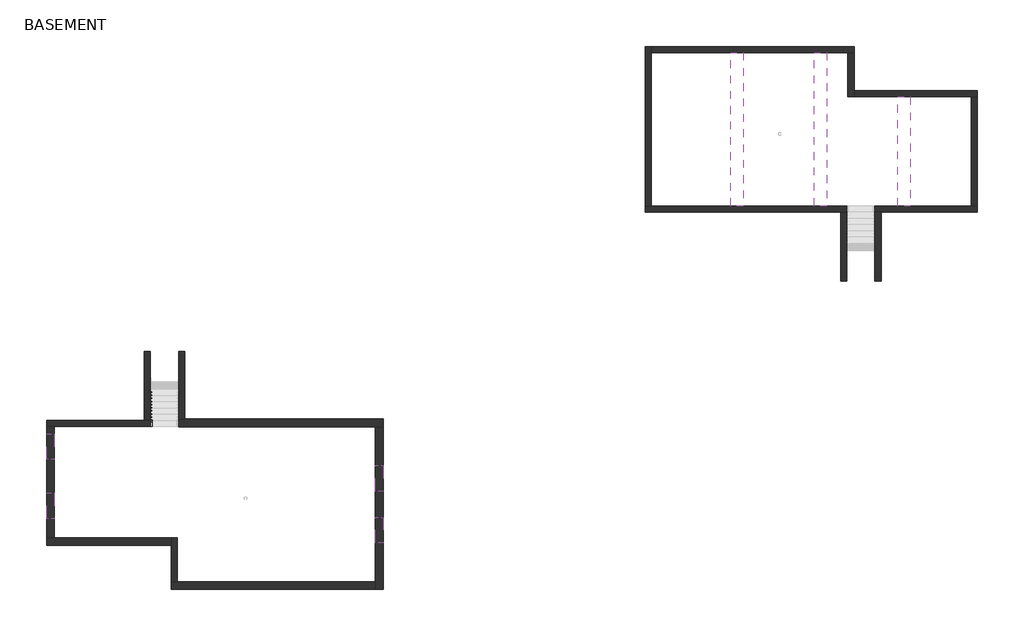
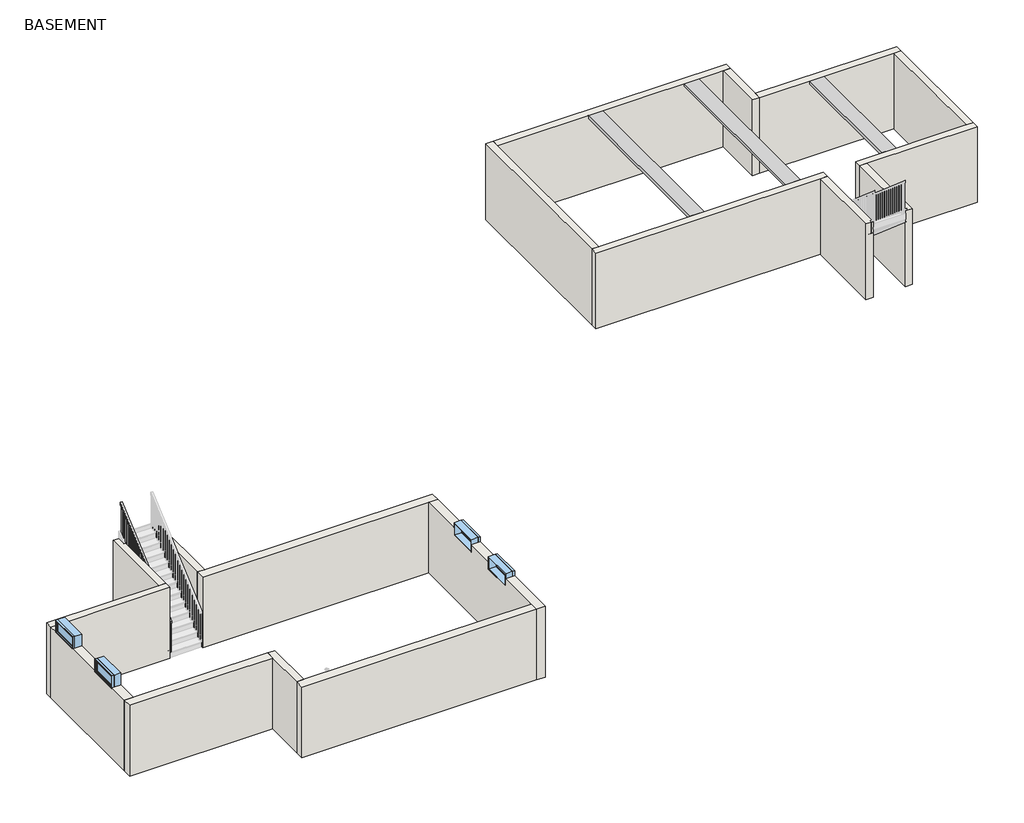
# One storey, part 1 of 2: 18 walls, 4 windows, 3 beams, 1 railing.
"""IFC4 building model written with IfcOpenShell, lengths in millimetres."""

import ifcopenshell
import ifcopenshell.guid

model = None  # the IFC model being written
_history = None  # IfcOwnerHistory: only IFC2X3 demands one
_inside = {}  # id of a spatial element -> (the spatial element, [elements in it])
_under = {}  # id of a project, library or spatial element -> (it, [spatial elements below it])
_declared = {}  # id of a project -> (the project, [libraries it declares])
_typed = {}  # id of a type object -> (the type object, [elements of that type])
_made_of = {}  # id of a material, layer set ... -> (it, [elements and type objects made of it])


def new_model(schema):
    """Start an empty IFC model of exactly this schema.

    Asked for "IFC4X3", IfcOpenShell would pick the latest addendum, in which some entities
    have other attributes; the version numbers below select the first issue.
    IFC2X3 requires an IfcOwnerHistory on every rooted entity: one is made here for all.
    """
    global model, _history
    if schema == "IFC4X3":
        model = ifcopenshell.file(schema_version=(4, 3, 0, 0))
    else:
        model = ifcopenshell.file(schema=schema)
    _inside.clear()
    _under.clear()
    _declared.clear()
    _typed.clear()
    _made_of.clear()
    _history = None
    if model.schema == "IFC2X3":
        org = make("IfcOrganization", Name="unknown")
        user = make(
            "IfcPersonAndOrganization",
            ThePerson=make("IfcPerson", FamilyName="unknown"),
            TheOrganization=org,
        )
        app = make(
            "IfcApplication",
            ApplicationDeveloper=org,
            Version="unknown",
            ApplicationFullName="unknown",
            ApplicationIdentifier="unknown",
        )
        _history = make(
            "IfcOwnerHistory",
            OwningUser=user,
            OwningApplication=app,
            ChangeAction="ADDED",
            CreationDate=0,
        )
    return model


def make(cls, **values):
    """One entity of the class cls with the attributes given. An attribute that is None is left unset."""
    return model.create_entity(
        cls, **{name: value for name, value in values.items() if value is not None}
    )


def rooted(cls, **values):
    """An entity with a GlobalId (a new one), such as an element, a storey or a relation."""
    return make(cls, GlobalId=ifcopenshell.guid.new(), OwnerHistory=_history, **values)


def si_unit(unit_type, name, prefix=None):
    """IfcSIUnit, for example si_unit("LENGTHUNIT", "METRE", prefix="MILLI")."""
    return make("IfcSIUnit", UnitType=unit_type, Prefix=prefix, Name=name)


def assignment(units):
    """IfcUnitAssignment: the units of a project."""
    return None if units is None else make("IfcUnitAssignment", Units=units)


def point(xyz):
    """IfcCartesianPoint."""
    return None if xyz is None else make("IfcCartesianPoint", Coordinates=xyz)


def direction(xyz):
    """IfcDirection."""
    return None if xyz is None else make("IfcDirection", DirectionRatios=xyz)


def frame(location, z_axis=None, x_axis=None):
    """IfcAxis2Placement3D, a coordinate frame: its origin and axes. An axis left out is left unset."""
    return make(
        "IfcAxis2Placement3D",
        Location=point(location),
        Axis=direction(z_axis),
        RefDirection=direction(x_axis),
    )


def origin():
    """The frame at (0, 0, 0) with its axes left unset."""
    return frame((0.0, 0.0, 0.0))


def place(relative_to, where):
    """IfcLocalPlacement: puts the frame where relative to a parent placement (None: the world)."""
    return make(
        "IfcLocalPlacement", PlacementRelTo=relative_to, RelativePlacement=where
    )


def context(
    kind, dimensions, precision=None, world=None, true_north=None, identifier=None
):
    """IfcGeometricRepresentationContext, for example the 3D "Model" context."""
    return make(
        "IfcGeometricRepresentationContext",
        ContextIdentifier=identifier,
        ContextType=kind,
        CoordinateSpaceDimension=dimensions,
        Precision=precision,
        WorldCoordinateSystem=world,
        TrueNorth=true_north,
    )


def project(units=None, contexts=None):
    """IfcProject with its units and contexts."""
    return rooted(
        "IfcProject",
        Name="project",
        RepresentationContexts=contexts,
        UnitsInContext=assignment(units),
    )


def spatial(cls, under=None, at=None, **own):
    """A site, building, storey or space (cls), placed at a placement, below another one or the project."""
    s = rooted(cls, ObjectPlacement=at, **own)
    if under is not None:
        _under.setdefault(under.id(), (under, []))[1].append(s)
    return s


def polyline(points):
    """IfcPolyline through the points."""
    return make("IfcPolyline", Points=[point(p) for p in points])


def outline(outer, holes=None, kind="AREA"):
    """IfcArbitraryClosedProfileDef: a profile drawn as a closed curve; with holes, ...WithVoids."""
    if holes is None:
        return make("IfcArbitraryClosedProfileDef", ProfileType=kind, OuterCurve=outer)
    return make(
        "IfcArbitraryProfileDefWithVoids",
        ProfileType=kind,
        OuterCurve=outer,
        InnerCurves=holes,
    )


def extrude(swept, where, along, depth):
    """IfcExtrudedAreaSolid: the profile swept, set in the frame where, extruded along a direction by depth."""
    return make(
        "IfcExtrudedAreaSolid",
        SweptArea=swept,
        Position=where,
        ExtrudedDirection=direction(along),
        Depth=depth,
    )


def faces_of(points, faces, orient=None, outer=None):
    """IfcFace entities. A face is a list of loops; a loop is a list of indices into points, from 0.

    orient and outer hold one flag for each loop. By default every Orientation is true, the
    first loop of a face is its IfcFaceOuterBound and the others are IfcFaceBound.
    """
    made = []
    for i, loops in enumerate(faces):
        bounds = []
        for j, loop in enumerate(loops):
            is_outer = j == 0 if outer is None else outer[i][j]
            bounds.append(
                make(
                    "IfcFaceOuterBound" if is_outer else "IfcFaceBound",
                    Bound=make("IfcPolyLoop", Polygon=[points[k] for k in loop]),
                    Orientation=True if orient is None else orient[i][j],
                )
            )
        made.append(make("IfcFace", Bounds=bounds))
    return made


def faceted_brep(points, faces, orient=None, outer=None, voids=None):
    """IfcFacetedBrep: a solid bounded by flat faces; with voids (closed shells), ...WithVoids."""
    shared = [point(p) for p in points]
    hull = make("IfcClosedShell", CfsFaces=faces_of(shared, faces, orient, outer))
    if voids is None:
        return make("IfcFacetedBrep", Outer=hull)
    return make(
        "IfcFacetedBrepWithVoids",
        Outer=hull,
        Voids=[
            make(cls, CfsFaces=faces_of(shared, fs, o, b)) for cls, fs, o, b in voids
        ],
    )


def shape(context_of_items, identifier, shape_type, items):
    """IfcShapeRepresentation: the items that make up one representation, for example the "Body"."""
    return make(
        "IfcShapeRepresentation",
        ContextOfItems=context_of_items,
        RepresentationIdentifier=identifier,
        RepresentationType=shape_type,
        Items=items,
    )


def source(mapping_origin, context_of_items, identifier, shape_type, items):
    """IfcRepresentationMap: a shape defined once, which mapped items show again and again."""
    return make(
        "IfcRepresentationMap",
        MappingOrigin=mapping_origin,
        MappedRepresentation=shape(context_of_items, identifier, shape_type, items),
    )


def transform(
    local_origin,
    x_axis=None,
    y_axis=None,
    z_axis=None,
    scale=None,
    scale2=None,
    scale3=None,
    uniform=True,
):
    """IfcCartesianTransformationOperator3D, or its non-uniform kind. x_axis, y_axis, z_axis: its Axis1, 2, 3."""
    if uniform:
        return make(
            "IfcCartesianTransformationOperator3D",
            Axis1=direction(x_axis),
            Axis2=direction(y_axis),
            LocalOrigin=point(local_origin),
            Scale=scale,
            Axis3=direction(z_axis),
        )
    return make(
        "IfcCartesianTransformationOperator3DnonUniform",
        Axis1=direction(x_axis),
        Axis2=direction(y_axis),
        LocalOrigin=point(local_origin),
        Scale=scale,
        Axis3=direction(z_axis),
        Scale2=scale2,
        Scale3=scale3,
    )


def mapped(mapping_source, mapping_target):
    """IfcMappedItem: shows the shape of a source again, moved by a transform."""
    return make(
        "IfcMappedItem", MappingSource=mapping_source, MappingTarget=mapping_target
    )


def made_of(thing, what):
    """Note that an element or type object is made of a material, layer set ...; save() writes the relation."""
    if what is not None:
        _made_of.setdefault(what.id(), (what, []))[1].append(thing)
    return thing


def element(
    cls,
    number,
    at=None,
    inside=None,
    cuts=None,
    type_object=None,
    material=None,
    context=None,
    identifier="Body",
    shape_type=None,
    held_by="IfcProductDefinitionShape",
    body=None,
    shapes=None,
    **own,
):
    """One element of the class cls, such as IfcWall. Its Tag is "e" and its number.

    at: its placement. inside: the storey or other place that contains it. cuts: it is an
    opening in that element (IfcRelVoidsElement). A single representation is given by context,
    identifier, shape_type and body (its items); several are given by shapes. held_by: the class
    of the entity that holds the representations. save() writes the other relations.
    """
    e = rooted(cls, Tag="e%d" % number, ObjectPlacement=at, **own)
    if body is not None:
        shapes = [shape(context, identifier, shape_type, body)]
    if shapes is not None:
        e.Representation = make(held_by, Representations=shapes)
    if inside is not None:
        _inside.setdefault(inside.id(), (inside, []))[1].append(e)
    if cuts is not None:
        rooted(
            "IfcRelVoidsElement", RelatingBuildingElement=cuts, RelatedOpeningElement=e
        )
    if type_object is not None:
        _typed.setdefault(type_object.id(), (type_object, []))[1].append(e)
    return made_of(e, material)


def aggregate(whole, parts):
    """IfcRelAggregates: a whole, such as a stair, and the parts it consists of."""
    return rooted("IfcRelAggregates", RelatingObject=whole, RelatedObjects=parts)


def save(model, path):
    """Write the relations noted so far, then the file.

    IfcRelAggregates (storeys below a building ...), IfcRelContainedInSpatialStructure (elements
    in a storey), IfcRelDefinesByType, IfcRelAssociatesMaterial and IfcRelDeclares: one each for
    every whole, place, type object, material and project.
    """
    for whole, parts in _under.values():
        aggregate(whole, parts)
    for where, things in _inside.values():
        rooted(
            "IfcRelContainedInSpatialStructure",
            RelatedElements=things,
            RelatingStructure=where,
        )
    for kind, things in _typed.values():
        rooted("IfcRelDefinesByType", RelatedObjects=things, RelatingType=kind)
    for what, things in _made_of.values():
        rooted("IfcRelAssociatesMaterial", RelatedObjects=things, RelatingMaterial=what)
    for by, libraries in _declared.values():
        rooted("IfcRelDeclares", RelatingContext=by, RelatedDefinitions=libraries)
    model.write(path)


def window_bf5cd34b(model_context):
    return source(origin(), model_context, "Body", "SweptSolid", [
        extrude(outline(polyline([(317.5, 79.375), (-393.7, 79.375), (-393.7, 92.075), (317.5, 92.075), (317.5, 79.375)])), frame((0.0, 0.0, 977.9), z_axis=(0.0, 0.0, 1.0), x_axis=(1.0, 0.0, 0.0)), (0.0, 0.0, 1.0), 254.0),
        extrude(outline(polyline([(1276.35, -438.15), (933.45, -438.15), (933.45, 361.95), (1276.35, 361.95), (1276.35, -438.15)]), holes=[polyline([(1231.9, -393.7), (1231.9, 317.5), (977.9, 317.5), (977.9, -393.7), (1231.9, -393.7)])]), frame((0.0, 63.5, 0.0), z_axis=(0.0, 1.0, 0.0), x_axis=(0.0, 0.0, 1.0)), (0.0, 0.0, 1.0), 44.45),
        extrude(outline(polyline([(1295.4, -457.2), (914.4, -457.2), (914.4, 381.0), (1295.4, 381.0), (1295.4, -457.2)]), holes=[polyline([(1263.65, -425.45), (1263.65, 349.25), (946.15, 349.25), (946.15, -425.45), (1263.65, -425.45)])]), frame((0.0, -127.0, 0.0), z_axis=(0.0, 1.0, 0.0), x_axis=(0.0, 0.0, 1.0)), (0.0, 0.0, 1.0), 190.5),
        extrude(outline(polyline([(1295.4, 381.0), (1295.4, -457.2), (914.4, -457.2), (914.4, 381.0), (1295.4, 381.0)]), holes=[polyline([(1276.35, 361.95), (933.45, 361.95), (933.45, -438.15), (1276.35, -438.15), (1276.35, 361.95)])]), frame((0.0, 63.5, 0.0), z_axis=(0.0, 1.0, 0.0), x_axis=(0.0, 0.0, 1.0)), (0.0, 0.0, 1.0), 63.5),
    ])


model = new_model("IFC4")

# Units and contexts
model_context = context("Model", 3, world=origin())
ifc_project = project(units=[si_unit("LENGTHUNIT", "METRE", prefix="MILLI")], contexts=[model_context])

# Site, building, storey
site = spatial("IfcSite", under=ifc_project)
building = spatial("IfcBuilding", under=site)
storey = spatial("IfcBuildingStorey", under=building, Name="BASEMENT", Elevation=-2266.95)

# Beams
placement = place(None, origin())
element("IfcBeam", 1, ObjectType="Concrete-Rectangular Beam : width=1' - 4\" x depth=0'  3 1/4\"", at=placement, inside=storey, context=model_context, shape_type="SweptSolid", body=[
    extrude(outline(polyline([(-3464.4595256, -410.4444564), (-3058.0595256, -410.4444564), (-3058.0595256, -5395.1944564), (-3464.4595256, -5395.1944564), (-3464.4595256, -410.4444564)])), frame((0.0, 0.0, -82.55), z_axis=(0.0, 0.0, 1.0), x_axis=(1.0, 0.0, 0.0)), (0.0, 0.0, 1.0), 82.55),
])
element("IfcBeam", 2, ObjectType="Concrete-Rectangular Beam : width=1' - 4\" x depth=0'  3 1/4\"", at=placement, inside=storey, context=model_context, shape_type="SweptSolid", body=[
    extrude(outline(polyline([(-6182.2595256, -410.4444564), (-5775.8595256, -410.4444564), (-5775.8595256, -5395.1944564), (-6182.2595256, -5395.1944564), (-6182.2595256, -410.4444564)])), frame((0.0, 0.0, -82.55), z_axis=(0.0, 0.0, 1.0), x_axis=(1.0, 0.0, 0.0)), (0.0, 0.0, 1.0), 82.55),
])
element("IfcBeam", 3, ObjectType="Concrete-Rectangular Beam : width=1' - 4\" x depth=0'  3 1/4\"", at=placement, inside=storey, context=model_context, shape_type="SweptSolid", body=[
    extrude(outline(polyline([(-746.6595256, -1845.5444564), (-340.2595256, -1845.5444564), (-340.2595256, -5395.1944564), (-746.6595256, -5395.1944564), (-746.6595256, -1845.5444564)])), frame((0.0, 0.0, -82.55), z_axis=(0.0, 0.0, 1.0), x_axis=(1.0, 0.0, 0.0)), (0.0, 0.0, 1.0), 82.55),
])

# Railing
element("IfcRailing", 4, ObjectType="Handrail - Rectangular", at=placement, inside=storey, context=model_context, shape_type="SweptSolid", body=[
    extrude(outline(polyline([(-12572.2570712, -1245.110853), (-12572.2570712, -1178.1692308), (-10133.8570712, 914.4), (-10133.8570712, 847.4583777), (-12572.2570712, -1245.110853)])), frame((-25042.4664763, 0.0, 0.0), z_axis=(1.0, 0.0, 0.0), x_axis=(0.0, 1.0, 0.0)), (0.0, 0.0, 1.0), 50.8),
    extrude(outline(polyline([(-10225.9320712, 768.4420917), (-10225.9320712, -174.3807692), (-10244.9820712, -174.3807692), (-10244.9820712, 752.0938946), (-10225.9320712, 768.4420917)])), frame((-25026.5914763, 0.0, 0.0), z_axis=(1.0, 0.0, 0.0), x_axis=(0.0, 1.0, 0.0)), (0.0, 0.0, 1.0), 19.05),
    extrude(outline(polyline([(-10327.5320712, 681.2517071), (-10327.5320712, -174.3807692), (-10346.5820712, -174.3807692), (-10346.5820712, 664.9035099), (-10327.5320712, 681.2517071)])), frame((-25026.5914763, 0.0, 0.0), z_axis=(1.0, 0.0, 0.0), x_axis=(0.0, 1.0, 0.0)), (0.0, 0.0, 1.0), 19.05),
    extrude(outline(polyline([(-10429.1320712, 594.0613224), (-10429.1320712, -348.7615385), (-10448.1820712, -348.7615385), (-10448.1820712, 577.7131253), (-10429.1320712, 594.0613224)])), frame((-25026.5914763, 0.0, 0.0), z_axis=(1.0, 0.0, 0.0), x_axis=(0.0, 1.0, 0.0)), (0.0, 0.0, 1.0), 19.05),
    extrude(outline(polyline([(-10530.7320712, 506.8709378), (-10530.7320712, -348.7615385), (-10549.7820712, -348.7615385), (-10549.7820712, 490.5227407), (-10530.7320712, 506.8709378)])), frame((-25026.5914763, 0.0, 0.0), z_axis=(1.0, 0.0, 0.0), x_axis=(0.0, 1.0, 0.0)), (0.0, 0.0, 1.0), 19.05),
    extrude(outline(polyline([(-10632.3320712, 419.6805532), (-10632.3320712, -523.1423077), (-10651.3820712, -523.1423077), (-10651.3820712, 403.3323561), (-10632.3320712, 419.6805532)])), frame((-25026.5914763, 0.0, 0.0), z_axis=(1.0, 0.0, 0.0), x_axis=(0.0, 1.0, 0.0)), (0.0, 0.0, 1.0), 19.05),
    extrude(outline(polyline([(-10733.9320712, 332.4901686), (-10733.9320712, -523.1423077), (-10752.9820712, -523.1423077), (-10752.9820712, 316.1419715), (-10733.9320712, 332.4901686)])), frame((-25026.5914763, 0.0, 0.0), z_axis=(1.0, 0.0, 0.0), x_axis=(0.0, 1.0, 0.0)), (0.0, 0.0, 1.0), 19.05),
    extrude(outline(polyline([(-10835.5320712, 245.299784), (-10835.5320712, -697.5230769), (-10854.5820712, -697.5230769), (-10854.5820712, 228.9515869), (-10835.5320712, 245.299784)])), frame((-25026.5914763, 0.0, 0.0), z_axis=(1.0, 0.0, 0.0), x_axis=(0.0, 1.0, 0.0)), (0.0, 0.0, 1.0), 19.05),
    extrude(outline(polyline([(-10937.1320712, 158.1093994), (-10937.1320712, -697.5230769), (-10956.1820712, -697.5230769), (-10956.1820712, 141.7612022), (-10937.1320712, 158.1093994)])), frame((-25026.5914763, 0.0, 0.0), z_axis=(1.0, 0.0, 0.0), x_axis=(0.0, 1.0, 0.0)), (0.0, 0.0, 1.0), 19.05),
    extrude(outline(polyline([(-11038.7320712, 70.9190147), (-11038.7320712, -871.9038462), (-11057.7820712, -871.9038462), (-11057.7820712, 54.5708176), (-11038.7320712, 70.9190147)])), frame((-25026.5914763, 0.0, 0.0), z_axis=(1.0, 0.0, 0.0), x_axis=(0.0, 1.0, 0.0)), (0.0, 0.0, 1.0), 19.05),
    extrude(outline(polyline([(-11140.3320712, -16.2713699), (-11140.3320712, -871.9038462), (-11159.3820712, -871.9038462), (-11159.3820712, -32.619567), (-11140.3320712, -16.2713699)])), frame((-25026.5914763, 0.0, 0.0), z_axis=(1.0, 0.0, 0.0), x_axis=(0.0, 1.0, 0.0)), (0.0, 0.0, 1.0), 19.05),
    extrude(outline(polyline([(-11241.9320712, -103.4617545), (-11241.9320712, -1046.2846154), (-11260.9820712, -1046.2846154), (-11260.9820712, -119.8099516), (-11241.9320712, -103.4617545)])), frame((-25026.5914763, 0.0, 0.0), z_axis=(1.0, 0.0, 0.0), x_axis=(0.0, 1.0, 0.0)), (0.0, 0.0, 1.0), 19.05),
    extrude(outline(polyline([(-11343.5320712, -190.6521391), (-11343.5320712, -1046.2846154), (-11362.5820712, -1046.2846154), (-11362.5820712, -207.0003362), (-11343.5320712, -190.6521391)])), frame((-25026.5914763, 0.0, 0.0), z_axis=(1.0, 0.0, 0.0), x_axis=(0.0, 1.0, 0.0)), (0.0, 0.0, 1.0), 19.05),
    extrude(outline(polyline([(-11445.1320712, -277.8425237), (-11445.1320712, -1220.6653846), (-11464.1820712, -1220.6653846), (-11464.1820712, -294.1907208), (-11445.1320712, -277.8425237)])), frame((-25026.5914763, 0.0, 0.0), z_axis=(1.0, 0.0, 0.0), x_axis=(0.0, 1.0, 0.0)), (0.0, 0.0, 1.0), 19.05),
    extrude(outline(polyline([(-11546.7320712, -365.0329083), (-11546.7320712, -1220.6653846), (-11565.7820712, -1220.6653846), (-11565.7820712, -381.3811054), (-11546.7320712, -365.0329083)])), frame((-25026.5914763, 0.0, 0.0), z_axis=(1.0, 0.0, 0.0), x_axis=(0.0, 1.0, 0.0)), (0.0, 0.0, 1.0), 19.05),
    extrude(outline(polyline([(-11648.3320712, -452.2232929), (-11648.3320712, -1395.0461538), (-11667.3820712, -1395.0461538), (-11667.3820712, -468.5714901), (-11648.3320712, -452.2232929)])), frame((-25026.5914763, 0.0, 0.0), z_axis=(1.0, 0.0, 0.0), x_axis=(0.0, 1.0, 0.0)), (0.0, 0.0, 1.0), 19.05),
    extrude(outline(polyline([(-11749.9320712, -539.4136776), (-11749.9320712, -1395.0461538), (-11768.9820712, -1395.0461538), (-11768.9820712, -555.7618747), (-11749.9320712, -539.4136776)])), frame((-25026.5914763, 0.0, 0.0), z_axis=(1.0, 0.0, 0.0), x_axis=(0.0, 1.0, 0.0)), (0.0, 0.0, 1.0), 19.05),
    extrude(outline(polyline([(-11851.5320712, -626.6040622), (-11851.5320712, -1569.4269231), (-11870.5820712, -1569.4269231), (-11870.5820712, -642.9522593), (-11851.5320712, -626.6040622)])), frame((-25026.5914763, 0.0, 0.0), z_axis=(1.0, 0.0, 0.0), x_axis=(0.0, 1.0, 0.0)), (0.0, 0.0, 1.0), 19.05),
    extrude(outline(polyline([(-11953.1320712, -713.7944468), (-11953.1320712, -1569.4269231), (-11972.1820712, -1569.4269231), (-11972.1820712, -730.1426439), (-11953.1320712, -713.7944468)])), frame((-25026.5914763, 0.0, 0.0), z_axis=(1.0, 0.0, 0.0), x_axis=(0.0, 1.0, 0.0)), (0.0, 0.0, 1.0), 19.05),
    extrude(outline(polyline([(-12054.7320712, -800.9848314), (-12054.7320712, -1743.8076923), (-12073.7820712, -1743.8076923), (-12073.7820712, -817.3330285), (-12054.7320712, -800.9848314)])), frame((-25026.5914763, 0.0, 0.0), z_axis=(1.0, 0.0, 0.0), x_axis=(0.0, 1.0, 0.0)), (0.0, 0.0, 1.0), 19.05),
    extrude(outline(polyline([(-12156.3320712, -888.175216), (-12156.3320712, -1743.8076923), (-12175.3820712, -1743.8076923), (-12175.3820712, -904.5234131), (-12156.3320712, -888.175216)])), frame((-25026.5914763, 0.0, 0.0), z_axis=(1.0, 0.0, 0.0), x_axis=(0.0, 1.0, 0.0)), (0.0, 0.0, 1.0), 19.05),
    extrude(outline(polyline([(-12257.9320712, -975.3656006), (-12257.9320712, -1918.1884615), (-12276.9820712, -1918.1884615), (-12276.9820712, -991.7137978), (-12257.9320712, -975.3656006)])), frame((-25026.5914763, 0.0, 0.0), z_axis=(1.0, 0.0, 0.0), x_axis=(0.0, 1.0, 0.0)), (0.0, 0.0, 1.0), 19.05),
    extrude(outline(polyline([(-12359.5320712, -1062.5559853), (-12359.5320712, -1918.1884615), (-12378.5820712, -1918.1884615), (-12378.5820712, -1078.9041824), (-12359.5320712, -1062.5559853)])), frame((-25026.5914763, 0.0, 0.0), z_axis=(1.0, 0.0, 0.0), x_axis=(0.0, 1.0, 0.0)), (0.0, 0.0, 1.0), 19.05),
    extrude(outline(polyline([(-12461.1320712, -1149.7463699), (-12461.1320712, -2092.5692308), (-12480.1820712, -2092.5692308), (-12480.1820712, -1166.094567), (-12461.1320712, -1149.7463699)])), frame((-25026.5914763, 0.0, 0.0), z_axis=(1.0, 0.0, 0.0), x_axis=(0.0, 1.0, 0.0)), (0.0, 0.0, 1.0), 19.05),
    extrude(outline(polyline([(-10133.8570712, 847.4583777), (-10133.8570712, -174.3807692), (-10152.9070712, -174.3807692), (-10152.9070712, 831.1101806), (-10133.8570712, 847.4583777)])), frame((-25026.5914763, 0.0, 0.0), z_axis=(1.0, 0.0, 0.0), x_axis=(0.0, 1.0, 0.0)), (0.0, 0.0, 1.0), 19.05),
    extrude(outline(polyline([(-12553.2070712, -1228.7626559), (-12553.2070712, -2092.5692308), (-12572.2570712, -2092.5692308), (-12572.2570712, -1245.110853), (-12553.2070712, -1228.7626559)])), frame((-25026.5914763, 0.0, 0.0), z_axis=(1.0, 0.0, 0.0), x_axis=(0.0, 1.0, 0.0)), (0.0, 0.0, 1.0), 19.05),
])

# Walls
element("IfcWall", 5, ObjectType="Generic - 10\"", at=placement, inside=storey, context=model_context, shape_type="Brep", body=[
    faceted_brep([(-17733.6164763, -12584.9570712, -2266.95), (-17733.6164763, -17620.5070712, -2266.95), (-17733.6164763, -17874.5070712, -2266.95), (-17733.6164763, -17874.5070712, -152.4), (-17733.6164763, -17620.5070712, -152.4), (-17733.6164763, -16361.0904046, -152.4), (-17733.6164763, -16361.0904046, -381.0), (-17733.6164763, -15522.8904046, -381.0), (-17733.6164763, -15522.8904046, -152.4), (-17733.6164763, -14682.5737379, -152.4), (-17733.6164763, -14682.5737379, -381.0), (-17733.6164763, -13844.3737379, -381.0), (-17733.6164763, -13844.3737379, -152.4), (-17733.6164763, -12584.9570712, -152.4), (-17479.6164763, -17874.5070712, -2266.95), (-17479.6164763, -12584.9570712, -2266.95), (-17479.6164763, -12584.9570712, -152.4), (-17479.6164763, -13844.3737379, -152.4), (-17479.6164763, -13844.3737379, -381.0), (-17479.6164763, -14682.5737379, -381.0), (-17479.6164763, -14682.5737379, -152.4), (-17479.6164763, -15522.8904046, -152.4), (-17479.6164763, -15522.8904046, -381.0), (-17479.6164763, -16361.0904046, -381.0), (-17479.6164763, -16361.0904046, -152.4), (-17479.6164763, -17874.5070712, -152.4)], [[[0, 1, 2, 3, 4, 5, 6, 7, 8, 9, 10, 11, 12, 13]], [[14, 15, 16, 17, 18, 19, 20, 21, 22, 23, 24, 25]], [[2, 1, 0, 15, 14]], [[0, 13, 16, 15]], [[3, 2, 14, 25]], [[3, 25, 24, 5, 4]], [[8, 21, 20, 9]], [[16, 13, 12, 17]], [[23, 6, 5, 24]], [[6, 23, 22, 7]], [[7, 22, 21, 8]], [[19, 10, 9, 20]], [[10, 19, 18, 11]], [[11, 18, 17, 12]]]),
])
element("IfcWall", 6, ObjectType="Generic - 10\"", at=placement, inside=storey, context=model_context, shape_type="Brep", body=[
    faceted_brep([(-17733.6164763, -17620.5070712, -2266.95), (-24172.5164763, -17620.5070712, -2266.95), (-24375.7164763, -17620.5070712, -2266.95), (-24375.7164763, -17620.5070712, -152.4), (-24172.5164763, -17620.5070712, -152.4), (-17733.6164763, -17620.5070712, -152.4), (-17733.6164763, -17874.5070712, -2266.95), (-17733.6164763, -17874.5070712, -152.4), (-24375.7164763, -17874.5070712, -152.4), (-24375.7164763, -17874.5070712, -2266.95)], [[[0, 1, 2, 3, 4, 5]], [[6, 7, 8, 9]], [[2, 1, 0, 6, 9]], [[0, 5, 7, 6]], [[3, 2, 9, 8]], [[5, 4, 3, 8, 7]]]),
])
element("IfcWall", 7, ObjectType="Generic - 10\"", at=placement, inside=storey, context=model_context, shape_type="Brep", body=[
    faceted_brep([(-24375.7164763, -16191.7570712, -2266.95), (-28173.0164763, -16191.7570712, -2266.95), (-28427.0164763, -16191.7570712, -2266.95), (-28427.0164763, -16191.7570712, -152.4), (-28173.0164763, -16191.7570712, -152.4), (-24375.7164763, -16191.7570712, -152.4), (-24375.7164763, -16445.7570712, -2266.95), (-24375.7164763, -16445.7570712, -152.4), (-25734.6164763, -16445.7570712, -152.4), (-28427.0164763, -16445.7570712, -152.4), (-28427.0164763, -16445.7570712, -2266.95)], [[[0, 1, 2, 3, 4, 5]], [[6, 7, 8, 9, 10]], [[2, 1, 0, 6, 10]], [[0, 5, 7, 6]], [[3, 2, 10, 9]], [[5, 4, 3, 9, 8, 7]]]),
])
element("IfcWall", 8, ObjectType="Generic - 10\"", at=placement, inside=storey, context=model_context, shape_type="SweptSolid", body=[
    extrude(outline(polyline([(-12572.2570712, -2266.95), (-16191.7570712, -2266.95), (-16191.7570712, -152.4), (-15575.8070712, -152.4), (-15575.8070712, -177.7746), (-14737.6070712, -177.7746), (-14737.6070712, -152.4), (-13651.7570712, -152.4), (-13651.7570712, -177.7746), (-12813.5570712, -177.7746), (-12813.5570712, -152.4), (-12572.2570712, -152.4), (-12572.2570712, -2266.95)])), frame((-28427.0164763, 0.0, 0.0), z_axis=(1.0, 0.0, 0.0), x_axis=(0.0, 1.0, 0.0)), (0.0, 0.0, 1.0), 254.0),
])
element("IfcWall", 9, ObjectType="Generic - 10\"", at=placement, inside=storey, context=model_context, shape_type="Brep", body=[
    faceted_brep([(-24134.4164763, -12584.9570712, -2266.95), (-17733.6164763, -12584.9570712, -2266.95), (-17479.6164763, -12584.9570712, -2266.95), (-17479.6164763, -12584.9570712, -152.4), (-17733.6164763, -12584.9570712, -152.4), (-24134.4164763, -12584.9570712, -152.4), (-24134.4164763, -12330.9570712, -2266.95), (-24134.4164763, -12330.9570712, -152.4), (-23931.2164763, -12330.9570712, -152.4), (-17479.6164763, -12330.9570712, -152.4), (-17479.6164763, -12330.9570712, -2266.95), (-23931.2164763, -12330.9570712, -2266.95)], [[[0, 1, 2, 3, 4, 5]], [[6, 7, 8, 9, 10, 11]], [[2, 1, 0, 6, 11, 10]], [[3, 2, 10, 9]], [[0, 5, 7, 6]], [[5, 4, 3, 9, 8, 7]]]),
])
element("IfcWall", 10, ObjectType="Generic - 8\"", at=placement, inside=storey, context=model_context, shape_type="Brep", body=[
    faceted_brep([(1844.1404744, -5395.1944564, -2266.95), (1640.9404744, -5395.1944564, -2266.95), (-1489.6095256, -5395.1944564, -2266.95), (-1489.6095256, -5395.1944564, 0.0), (1640.9404744, -5395.1944564, 0.0), (1844.1404744, -5395.1944564, 0.0), (1844.1404744, -5598.3944564, -2266.95), (1844.1404744, -5598.3944564, 0.0), (-1286.4095256, -5598.3944564, 0.0), (-1489.6095256, -5598.3944564, 0.0), (-1489.6095256, -5598.3944564, -2266.95), (-1286.4095256, -5598.3944564, -2266.95)], [[[0, 1, 2, 3, 4, 5]], [[6, 7, 8, 9, 10, 11]], [[2, 1, 0, 6, 11, 10]], [[5, 4, 3, 9, 8, 7]], [[0, 5, 7, 6]], [[3, 2, 10, 9]]]),
])
element("IfcWall", 11, ObjectType="Generic - 8\"", at=placement, inside=storey, context=model_context, shape_type="Brep", body=[
    faceted_brep([(-8760.3595256, -5395.1944564, -2266.95), (-8760.3595256, -410.4444564, -2266.95), (-8760.3595256, -207.2444564, -2266.95), (-8760.3595256, -207.2444564, 0.0), (-8760.3595256, -410.4444564, 0.0), (-8760.3595256, -5395.1944564, 0.0), (-8963.5595256, -5395.1944564, -2266.95), (-8963.5595256, -5395.1944564, 0.0), (-8963.5595256, -207.2444564, 0.0), (-8963.5595256, -207.2444564, -2266.95)], [[[0, 1, 2, 3, 4, 5]], [[6, 7, 8, 9]], [[2, 1, 0, 6, 9]], [[5, 4, 3, 8, 7]], [[0, 5, 7, 6]], [[3, 2, 9, 8]]]),
])
element("IfcWall", 12, ObjectType="Generic - 8\"", at=placement, inside=storey, context=model_context, shape_type="Brep", body=[
    faceted_brep([(-8760.3595256, -410.4444564, -2266.95), (-2365.9095256, -410.4444564, -2266.95), (-2162.7095256, -410.4444564, -2266.95), (-2162.7095256, -410.4444564, 0.0), (-2365.9095256, -410.4444564, 0.0), (-8760.3595256, -410.4444564, 0.0), (-8760.3595256, -207.2444564, -2266.95), (-8760.3595256, -207.2444564, 0.0), (-2162.7095256, -207.2444564, 0.0), (-2162.7095256, -207.2444564, -2266.95)], [[[0, 1, 2, 3, 4, 5]], [[6, 7, 8, 9]], [[2, 1, 0, 6, 9]], [[5, 4, 3, 8, 7]], [[0, 5, 7, 6]], [[3, 2, 9, 8]]]),
])
element("IfcWall", 13, ObjectType="Generic - 8\"", at=placement, inside=storey, context=model_context, shape_type="Brep", body=[
    faceted_brep([(-2365.9095256, -410.4444564, -2266.95), (-2365.9095256, -1845.5444564, -2266.95), (-2365.9095256, -1845.5444564, 0.0), (-2365.9095256, -410.4444564, 0.0), (-2162.7095256, -410.4444564, -2266.95), (-2162.7095256, -410.4444564, 0.0), (-2162.7095256, -1642.3444564, 0.0), (-2162.7095256, -1845.5444564, 0.0), (-2162.7095256, -1845.5444564, -2266.95), (-2162.7095256, -1642.3444564, -2266.95)], [[[0, 1, 2, 3]], [[4, 5, 6, 7, 8, 9]], [[1, 0, 4, 9, 8]], [[3, 2, 7, 6, 5]], [[0, 3, 5, 4]], [[2, 1, 8, 7]]]),
])
element("IfcWall", 14, ObjectType="Generic - 8\"", at=placement, inside=storey, context=model_context, shape_type="Brep", body=[
    faceted_brep([(-2162.7095256, -1845.5444564, -2266.95), (1640.9404744, -1845.5444564, -2266.95), (1844.1404744, -1845.5444564, -2266.95), (1844.1404744, -1845.5444564, 0.0), (1640.9404744, -1845.5444564, 0.0), (-2162.7095256, -1845.5444564, 0.0), (-2162.7095256, -1642.3444564, -2266.95), (-2162.7095256, -1642.3444564, 0.0), (1844.1404744, -1642.3444564, 0.0), (1844.1404744, -1642.3444564, -2266.95)], [[[0, 1, 2, 3, 4, 5]], [[6, 7, 8, 9]], [[2, 1, 0, 6, 9]], [[5, 4, 3, 8, 7]], [[0, 5, 7, 6]], [[3, 2, 9, 8]]]),
])
element("IfcWall", 15, ObjectType="Generic - 8\"", at=placement, inside=storey, context=model_context, shape_type="SweptSolid", body=[
    extrude(outline(polyline([(1640.9404744, -5395.1944564), (1640.9404744, -1845.5444564), (1844.1404744, -1845.5444564), (1844.1404744, -5395.1944564), (1640.9404744, -5395.1944564)])), frame((0.0, 0.0, -2266.95), z_axis=(0.0, 0.0, 1.0), x_axis=(1.0, 0.0, 0.0)), (0.0, 0.0, 1.0), 2266.95),
])
element("IfcWall", 16, ObjectType="Generic - 8\"", at=placement, inside=storey, context=model_context, shape_type="Brep", body=[
    faceted_brep([(-2404.0095256, -5395.1944564, -2266.95), (-8760.3595256, -5395.1944564, -2266.95), (-8963.5595256, -5395.1944564, -2266.95), (-8963.5595256, -5395.1944564, 0.0), (-8760.3595256, -5395.1944564, 0.0), (-2404.0095256, -5395.1944564, 0.0), (-2404.0095256, -5598.3944564, -2266.95), (-2404.0095256, -5598.3944564, 0.0), (-2607.2095256, -5598.3944564, 0.0), (-8963.5595256, -5598.3944564, 0.0), (-8963.5595256, -5598.3944564, -2266.95), (-2607.2095256, -5598.3944564, -2266.95)], [[[0, 1, 2, 3, 4, 5]], [[6, 7, 8, 9, 10, 11]], [[2, 1, 0, 6, 11, 10]], [[5, 4, 3, 9, 8, 7]], [[3, 2, 10, 9]], [[0, 5, 7, 6]]]),
])
element("IfcWall", 17, ObjectType="Generic - 8\"", at=placement, inside=storey, context=model_context, shape_type="SweptSolid", body=[
    extrude(outline(polyline([(-1489.6095256, -7833.5944564), (-1489.6095256, -5598.3944564), (-1286.4095256, -5598.3944564), (-1286.4095256, -7833.5944564), (-1489.6095256, -7833.5944564)])), frame((0.0, 0.0, -2266.95), z_axis=(0.0, 0.0, 1.0), x_axis=(1.0, 0.0, 0.0)), (0.0, 0.0, 1.0), 2266.95),
])
element("IfcWall", 18, ObjectType="Generic - 8\"", at=placement, inside=storey, context=model_context, shape_type="SweptSolid", body=[
    extrude(outline(polyline([(-2404.0095256, -5598.3944564), (-2404.0095256, -7833.5944564), (-2607.2095256, -7833.5944564), (-2607.2095256, -5598.3944564), (-2404.0095256, -5598.3944564)])), frame((0.0, 0.0, -2266.95), z_axis=(0.0, 0.0, 1.0), x_axis=(1.0, 0.0, 0.0)), (0.0, 0.0, 1.0), 2266.95),
])
element("IfcWall", 19, ObjectType="Generic - 8\"", at=placement, inside=storey, context=model_context, shape_type="Brep", body=[
    faceted_brep([(-28427.0164763, -12572.2570712, -2266.95), (-28173.0164763, -12572.2570712, -2266.95), (-25048.8164763, -12572.2570712, -2266.95), (-25048.8164763, -12572.2570712, -152.4), (-28173.0164763, -12572.2570712, -152.4), (-28427.0164763, -12572.2570712, -152.4), (-28427.0164763, -12369.0570712, -2266.95), (-28427.0164763, -12369.0570712, -152.4), (-25252.0164763, -12369.0570712, -152.4), (-25048.8164763, -12369.0570712, -152.4), (-25048.8164763, -12369.0570712, -2266.95), (-25252.0164763, -12369.0570712, -2266.95)], [[[0, 1, 2, 3, 4, 5]], [[6, 7, 8, 9, 10, 11]], [[2, 1, 0, 6, 11, 10]], [[0, 5, 7, 6]], [[3, 2, 10, 9]], [[5, 4, 3, 9, 8, 7]]]),
])
element("IfcWall", 20, ObjectType="Generic - 8\"", at=placement, inside=storey, context=model_context, shape_type="Brep", body=[
    faceted_brep([(-24172.5164763, -17620.5070712, -2266.95), (-24172.5164763, -16191.7570712, -2266.95), (-24172.5164763, -16191.7570712, -152.4), (-24172.5164763, -17620.5070712, -152.4), (-24375.7164763, -17620.5070712, -2266.95), (-24375.7164763, -17620.5070712, -152.4), (-24375.7164763, -16445.7570712, -152.4), (-24375.7164763, -16191.7570712, -152.4), (-24375.7164763, -16191.7570712, -2266.95), (-24375.7164763, -16445.7570712, -2266.95)], [[[0, 1, 2, 3]], [[4, 5, 6, 7, 8, 9]], [[1, 0, 4, 9, 8]], [[0, 3, 5, 4]], [[2, 1, 8, 7]], [[3, 2, 7, 6, 5]]]),
])
element("IfcWall", 21, ObjectType="Generic - 8\"", at=placement, inside=storey, context=model_context, shape_type="SweptSolid", body=[
    extrude(outline(polyline([(-25048.8164763, -10133.8570712), (-25048.8164763, -12369.0570712), (-25252.0164763, -12369.0570712), (-25252.0164763, -10133.8570712), (-25048.8164763, -10133.8570712)])), frame((0.0, 0.0, -2266.95), z_axis=(0.0, 0.0, 1.0), x_axis=(1.0, 0.0, 0.0)), (0.0, 0.0, 1.0), 2114.55),
])
element("IfcWall", 22, ObjectType="Generic - 8\"", at=placement, inside=storey, context=model_context, shape_type="SweptSolid", body=[
    extrude(outline(polyline([(-24134.4164763, -12330.9570712), (-24134.4164763, -10133.8570712), (-23931.2164763, -10133.8570712), (-23931.2164763, -12330.9570712), (-24134.4164763, -12330.9570712)])), frame((0.0, 0.0, -2266.95), z_axis=(0.0, 0.0, 1.0), x_axis=(1.0, 0.0, 0.0)), (0.0, 0.0, 1.0), 2114.55),
])

# Windows
window_shape = window_bf5cd34b(model_context)
element("IfcWindow", 23, ObjectType="Fixed : 2'-9\" x 1'-3\"", at=placement, inside=storey, context=model_context, shape_type="MappedRepresentation", body=[
    mapped(window_shape, transform((-28300.0164763, -15118.6070712, -1092.1746), x_axis=(0.0, 1.0, 0.0), y_axis=(-1.0, 0.0, 0.0), z_axis=(0.0, 0.0, 1.0))),
])
element("IfcWindow", 24, ObjectType="Fixed : 2'-9\" x 1'-3\"", at=placement, inside=storey, context=model_context, shape_type="MappedRepresentation", body=[
    mapped(window_shape, transform((-28300.0164763, -13194.5570712, -1092.1746), x_axis=(0.0, 1.0, 0.0), y_axis=(-1.0, 0.0, 0.0), z_axis=(0.0, 0.0, 1.0))),
])
element("IfcWindow", 25, ObjectType="Fixed : 2'-9\" x 1'-3\"", at=placement, inside=storey, context=model_context, shape_type="MappedRepresentation", body=[
    mapped(window_shape, transform((-17606.6164763, -14301.5737379, -1295.4), x_axis=(0.0, -1.0, 0.0), y_axis=(1.0, 0.0, 0.0), z_axis=(0.0, 0.0, 1.0))),
])
element("IfcWindow", 26, ObjectType="Fixed : 2'-9\" x 1'-3\"", at=placement, inside=storey, context=model_context, shape_type="MappedRepresentation", body=[
    mapped(window_shape, transform((-17606.6164763, -15980.0904046, -1295.4), x_axis=(0.0, -1.0, 0.0), y_axis=(1.0, 0.0, 0.0), z_axis=(0.0, 0.0, 1.0))),
])

save(model, "model.ifc")

# Revit data of these elements
# Project information
#   Project Issue Date = "Issue Date"
#   Project Status = "Project Status"
#   Client Name = "Owner"
#   Project Address = "Enter address here"
#   Project Name = "Project Name"
#   Project Number = "Project Number"
# Grids (mm)
#   "B": line (-20559.366, -20036.147) -> (-20559.366, -11545.141)
#   "C": line (-23277.166, -20036.147) -> (-23277.166, -11545.141)
#   "D": line (-25994.966, -20036.147) -> (-25994.966, -11545.141)
#   "1": line (-5979.06, 2068.696) -> (-5979.06, -6422.311)
#   "2": line (-3261.26, 2068.696) -> (-3261.26, -6422.311)
#   "3": line (-543.46, 2068.696) -> (-543.46, -6422.311)
# Type "Concrete-Rectangular Beam : width=1' - 4\" x depth=0'  3 1/4\""
#   Assembly Code = "B10"
#   Length [instance default] = 5' - 0"
#   b = 1' - 4"
#   h = 0' - 3 1/4"
#   Structural Material [instance default] = Concrete, Cast-in-Place gray
# Type "Handrail - Rectangular"
#   Assembly Code = "C2010400"
#   built-in parameter 1008612 = 0.0416667 (stored number, unit not read)
#   built-in parameter 1008611 = 0.0416667 (stored number, unit not read)
#   built-in parameter 1008609 = 0.333333 (stored number, unit not read)
#   built-in parameter 1008604 = 0.166667 (stored number, unit not read)
#   built-in parameter 1008603 = 0.166667 (stored number, unit not read)
#   Railing Height = 3' - 0"
#   built-in parameter 1008630 = 2
#   built-in parameter 1008610 = 2
#   built-in parameter 1008618 = Baluster - Square : 3/4"
# Type "Generic - 10\""
#   Assembly Code = "B2010"
#   Layers, outside or top first: 0' - 10" no material (function 1)
# Type "Generic - 8\""
#   Assembly Code = "B2010"
#   Layers, outside or top first: 0' - 8" no material (function 1)
# Type "Fixed : 2'-9\" x 1'-3\""
#   Type Mark = "29"
#   Construction Type Id = "GSP4R"
#   Assembly Code = "B2020100"
#   Analytic Construction = "1/8 in Pilkington single glazing"
#   Visual Light Transmittance = 0.9
#   Solar Heat Gain Coefficient = 0.78
#   Heat Transfer Coefficient (U) = 3.6886 W/(m²·K)
#   Height = 1' - 3"
#   Default Sill Height = 3' - 0"
#   Width = 2' - 9"
#   Window Inset = 0' - 0 3/4"
#   Glass Pane Material = Glass
#   Sash Material = Sash
#   Wall Closure = (empty or 0)
# Element 1 (IfcBeam, "Concrete-Rectangular Beam : width=1' - 4\" x depth=0'  3 1/4\"")
#   Structural Material = Concrete, Cast-in-Place gray
#   Phase Created = New Construction
#   Materials on its faces: "Concrete, Cast-in-Place gray"
# Elements 2, 3 (IfcBeam, "Concrete-Rectangular Beam : width=1' - 4\" x depth=0'  3 1/4\"")
#   Comments = ""
#   Structural Material = Concrete, Cast-in-Place gray
#   Phase Created = New Construction
#   Materials on its faces: "Concrete, Cast-in-Place gray"
# Element 4 (IfcRailing, "Handrail - Rectangular")
#   Phase Created = New Construction
# Elements 5, 6, 7, 8, 9 (IfcWall, "Generic - 10\"")
#   Top Offset = 0' - 0"
#   Base Offset = 0' - 0"
#   wall height = 6' - 11 1/4"
#   Phase Created = New Construction
#   Base Constraint = BASEMENT
#   Top Constraint = LEVEL 1
#   Materials on its faces: "Default Wall"
# Elements 10, 11, 12, 13, 14, 15, 16, 17, 18 (IfcWall, "Generic - 8\"")
#   Top Offset = 0' - 0"
#   Base Offset = 0' - 0"
#   wall height = 7' - 5 1/4"
#   Phase Created = New Construction
#   Base Constraint = BASEMENT
#   Top Constraint = LEVEL 1
#   Materials on its faces: "Default Wall"
# Elements 19, 20, 21, 22 (IfcWall, "Generic - 8\"")
#   Top Offset = 0' - 0"
#   Base Offset = 0' - 0"
#   wall height = 6' - 11 1/4"
#   Phase Created = New Construction
#   Base Constraint = BASEMENT
#   Top Constraint = LEVEL 1
#   Materials on its faces: "Default Wall"
# Element 23 (IfcWindow, "Fixed : 2'-9\" x 1'-3\"")
#   Mark = "26"
#   Phase Created = New Construction
#   Materials on its faces: "Sash", "Glass"
# Element 24 (IfcWindow, "Fixed : 2'-9\" x 1'-3\"")
#   Mark = "27"
#   Phase Created = New Construction
#   Materials on its faces: "Sash", "Glass"
# Element 25 (IfcWindow, "Fixed : 2'-9\" x 1'-3\"")
#   Mark = "28"
#   Phase Created = New Construction
#   Materials on its faces: "Sash", "Glass"
# Element 26 (IfcWindow, "Fixed : 2'-9\" x 1'-3\"")
#   Mark = "29"
#   Phase Created = New Construction
#   Materials on its faces: "Sash", "Glass"
# Materials
#   "Concrete, Cast-in-Place gray": class "Concrete", colour RGB 192 192 192, transparency 0, Description = "Cast-in-place concrete", Cost = 0
#   "Glass": class "Glass", colour RGB 0 128 192, transparency 0.75, Description = "Soda Lime Glass", Cost = 0
#   "Sash": class "Wood", colour RGB 224 178 126, transparency 0, Cost = 0
#   "Default Wall": class "Miscellaneous", colour RGB 128 128 128, transparency 0, Cost = 0
